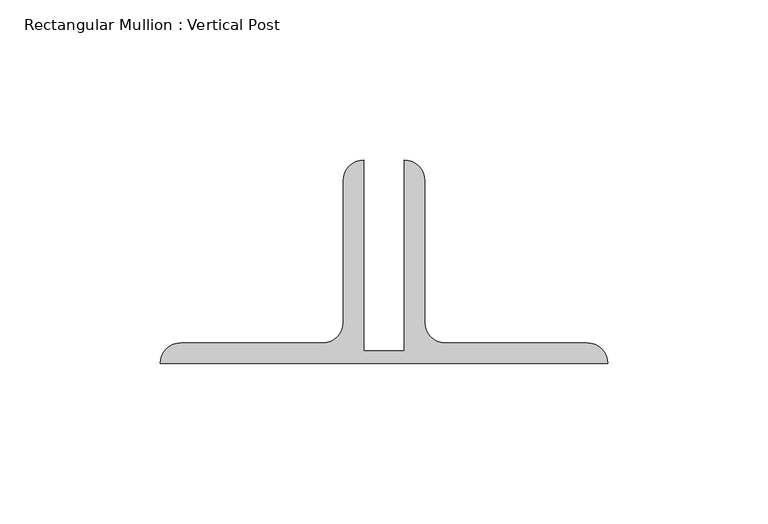
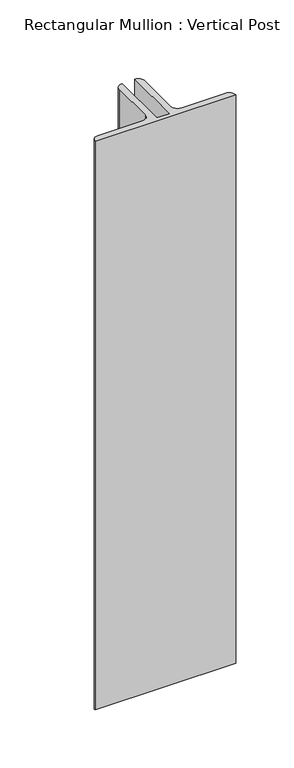
"""IFC4 building model written with IfcOpenShell, lengths in millimetres: member geometry, Rectangular Mullion : Vertical Post."""

from ifc_helpers import new_model, si_unit, point, frame, frame_2d, origin, place, context, project, spatial, polyline, circle_curve, trimmed, segment, composite_curve, outline, extrude, source, transform, mapped, element, save


def rectangular_mullion_vertical_post_f660218a(model_context):
    return source(origin(), model_context, "Body", "SweptSolid", [
        extrude(outline(composite_curve([segment(polyline([(-76.2, 22.9145205), (-63.5, 22.9145205), (-63.5, 82.55)]), True, "CONTINUOUS"), segment(trimmed(circle_curve(frame_2d((-63.5, 76.2)), 6.35), [point((-63.5, 82.55))], [point((-57.15, 76.2))], False, "CARTESIAN"), True, "CONTINUOUS"), segment(polyline([(-57.15, 76.2), (-57.15, 31.75)]), True, "CONTINUOUS"), segment(trimmed(circle_curve(frame_2d((-50.8, 31.75)), 6.35), [point((-57.15, 31.75))], [point((-50.8, 25.4))], True, "CARTESIAN"), True, "CONTINUOUS"), segment(polyline([(-50.8, 25.4), (-6.35, 25.4)]), True, "CONTINUOUS"), segment(trimmed(circle_curve(frame_2d((-6.35, 19.05)), 6.35), [point((-6.35, 25.4))], [point((0.0, 19.05))], False, "CARTESIAN"), True, "CONTINUOUS"), segment(polyline([(0.0, 19.05), (-139.7, 19.05)]), True, "CONTINUOUS"), segment(trimmed(circle_curve(frame_2d((-133.35, 19.05)), 6.35), [point((-139.7, 19.05))], [point((-133.35, 25.4))], False, "CARTESIAN"), True, "CONTINUOUS"), segment(polyline([(-133.35, 25.4), (-88.9, 25.4)]), True, "CONTINUOUS"), segment(trimmed(circle_curve(frame_2d((-88.9, 31.75)), 6.35), [point((-88.9, 25.4))], [point((-82.55, 31.75))], True, "CARTESIAN"), True, "CONTINUOUS"), segment(polyline([(-82.55, 31.75), (-82.55, 76.2)]), True, "CONTINUOUS"), segment(trimmed(circle_curve(frame_2d((-76.2, 76.2)), 6.35), [point((-82.55, 76.2))], [point((-76.2, 82.55))], False, "CARTESIAN"), True, "CONTINUOUS"), segment(polyline([(-76.2, 82.55), (-76.2, 22.9145205)]), True, "CONTINUOUS")], self_intersect=False)), frame((0.0, 0.0, -596.9), z_axis=(0.0, 0.0, 1.0), x_axis=(1.0, 0.0, 0.0)), (0.0, 0.0, 1.0), 596.9),
    ])


if __name__ == "__main__":
    model = new_model("IFC4")
    model_context = context("Model", 3, world=origin())
    ifc_project = project(units=[si_unit("LENGTHUNIT", "METRE", prefix="MILLI")], contexts=[model_context])
    site = spatial("IfcSite", under=ifc_project)
    building = spatial("IfcBuilding", under=site)
    placement = place(None, origin())
    rectangular_mullion_vertical_post_shape = rectangular_mullion_vertical_post_f660218a(model_context)
    element("IfcMember", 1, ObjectType="Rectangular Mullion : Vertical Post", at=placement, inside=building, context=model_context, shape_type="MappedRepresentation", body=[
        mapped(rectangular_mullion_vertical_post_shape, transform((0.0, 0.0, 0.0), x_axis=(1.0, 0.0, 0.0), y_axis=(0.0, 1.0, 0.0), z_axis=(0.0, 0.0, 1.0))),
    ])
    save(model, "model.ifc")

# Revit data of these elements
# Type "Rectangular Mullion : Vertical Post"
#   built-in parameter 1007351 = -0.0625 (stored number, unit not read)
#   built-in parameter 1007322 = 0.0126789 (stored number, unit not read)
#   built-in parameter 1007321 = 0.229167 (stored number, unit not read)
#   built-in parameter 1007320 = 0.229167 (stored number, unit not read)
# Element 1 (IfcMember, "Rectangular Mullion : Vertical Post")
#   Materials on its faces: "GATE POST: (2) BACK/BACK GALVANIZED ANGLES"
# Materials
#   "GATE POST: (2) BACK/BACK GALVANIZED ANGLES": class "Unassigned", colour RGB 211 211 211, transparency 0, Cost = 0
